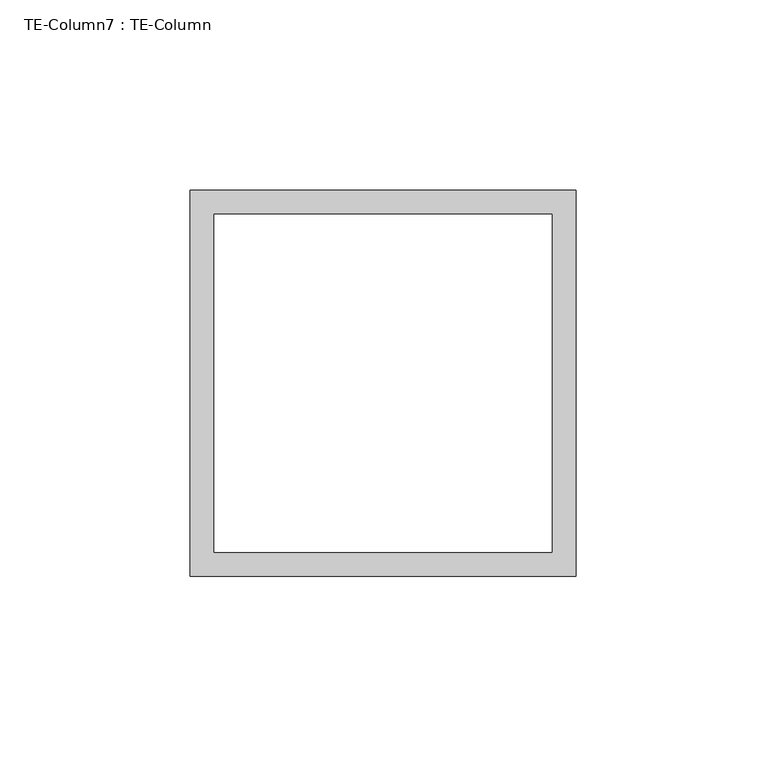
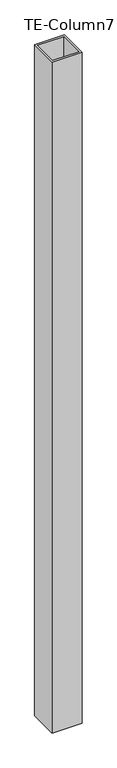
"""IFC4 building model written with IfcOpenShell, lengths in millimetres: proxy geometry, TE-Column7 : TE-Column."""

from ifc_helpers import new_model, si_unit, frame, origin, place, context, project, spatial, polyline, outline, extrude, source, transform, mapped, element, save


def te_column7_te_column_a47af242(model_context):
    return source(origin(), model_context, "Body", "SweptSolid", [
        extrude(outline(polyline([(590318.6434739, -536417.5913841), (590217.0434739, -536417.5913841), (590217.0434739, -536315.9913841), (590318.6434739, -536315.9913841), (590318.6434739, -536417.5913841)]), holes=[polyline([(590312.2934739, -536322.3413841), (590223.3934739, -536322.3413841), (590223.3934739, -536411.2413841), (590312.2934739, -536411.2413841), (590312.2934739, -536322.3413841)])]), frame((0.0, 0.0, 28.575), z_axis=(0.0, 0.0, 1.0), x_axis=(1.0, 0.0, 0.0)), (0.0, 0.0, 1.0), 2406.65),
    ])


if __name__ == "__main__":
    model = new_model("IFC4")
    model_context = context("Model", 3, world=origin())
    ifc_project = project(units=[si_unit("LENGTHUNIT", "METRE", prefix="MILLI")], contexts=[model_context])
    site = spatial("IfcSite", under=ifc_project)
    building = spatial("IfcBuilding", under=site)
    placement = place(None, origin())
    te_column7_te_column_shape = te_column7_te_column_a47af242(model_context)
    element("IfcBuildingElementProxy", 1, Name="TE-Column7 : TE-Column", ObjectType="TE-Column7 : TE-Column", at=placement, inside=building, context=model_context, shape_type="MappedRepresentation", body=[
        mapped(te_column7_te_column_shape, transform((0.0, 0.0, 0.0), x_axis=(1.0, 0.0, 0.0), y_axis=(0.0, 1.0, 0.0), z_axis=(0.0, 0.0, 1.0))),
    ])
    save(model, "model.ifc")

# Revit data of these elements
# Element 1 (IfcBuildingElementProxy, "TE-Column7 : TE-Column")
#   Materials on its faces: "4\"X4\" GALV. HSS TUBING"
# Materials
#   "4\"X4\" GALV. HSS TUBING": class "Generic", colour RGB 211 211 207, transparency 0, Cost = 0
